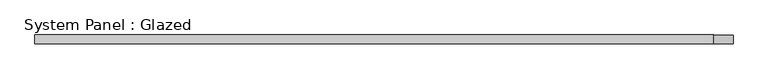
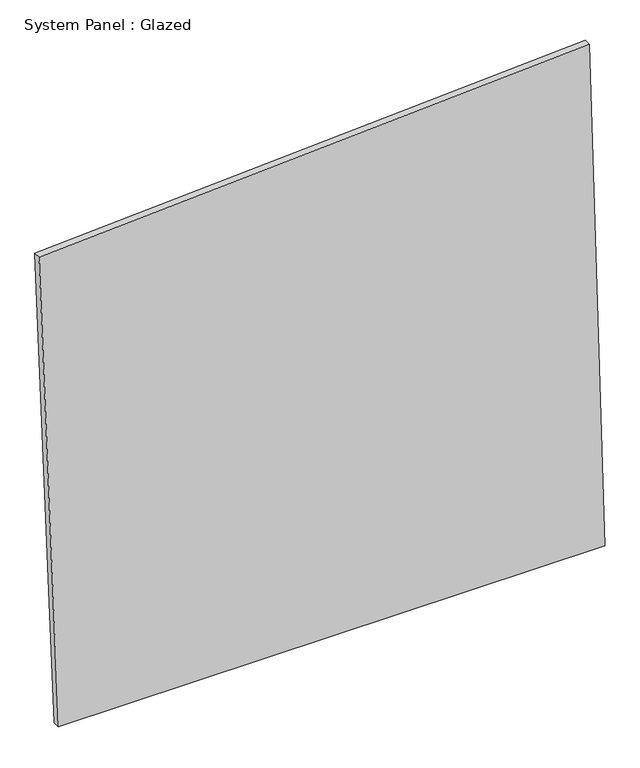
"""IFC4 building model written with IfcOpenShell, lengths in millimetres: plate geometry, System Panel : Glazed."""

import ifcopenshell
import ifcopenshell.guid

model = None  # the IFC model being written
_history = None  # IfcOwnerHistory: only IFC2X3 demands one
_inside = {}  # id of a spatial element -> (the spatial element, [elements in it])
_under = {}  # id of a project, library or spatial element -> (it, [spatial elements below it])
_declared = {}  # id of a project -> (the project, [libraries it declares])
_typed = {}  # id of a type object -> (the type object, [elements of that type])
_made_of = {}  # id of a material, layer set ... -> (it, [elements and type objects made of it])


def new_model(schema):
    """Start an empty IFC model of exactly this schema.

    Asked for "IFC4X3", IfcOpenShell would pick the latest addendum, in which some entities
    have other attributes; the version numbers below select the first issue.
    IFC2X3 requires an IfcOwnerHistory on every rooted entity: one is made here for all.
    """
    global model, _history
    if schema == "IFC4X3":
        model = ifcopenshell.file(schema_version=(4, 3, 0, 0))
    else:
        model = ifcopenshell.file(schema=schema)
    _inside.clear()
    _under.clear()
    _declared.clear()
    _typed.clear()
    _made_of.clear()
    _history = None
    if model.schema == "IFC2X3":
        org = make("IfcOrganization", Name="unknown")
        user = make(
            "IfcPersonAndOrganization",
            ThePerson=make("IfcPerson", FamilyName="unknown"),
            TheOrganization=org,
        )
        app = make(
            "IfcApplication",
            ApplicationDeveloper=org,
            Version="unknown",
            ApplicationFullName="unknown",
            ApplicationIdentifier="unknown",
        )
        _history = make(
            "IfcOwnerHistory",
            OwningUser=user,
            OwningApplication=app,
            ChangeAction="ADDED",
            CreationDate=0,
        )
    return model


def make(cls, **values):
    """One entity of the class cls with the attributes given. An attribute that is None is left unset."""
    return model.create_entity(
        cls, **{name: value for name, value in values.items() if value is not None}
    )


def rooted(cls, **values):
    """An entity with a GlobalId (a new one), such as an element, a storey or a relation."""
    return make(cls, GlobalId=ifcopenshell.guid.new(), OwnerHistory=_history, **values)


def si_unit(unit_type, name, prefix=None):
    """IfcSIUnit, for example si_unit("LENGTHUNIT", "METRE", prefix="MILLI")."""
    return make("IfcSIUnit", UnitType=unit_type, Prefix=prefix, Name=name)


def assignment(units):
    """IfcUnitAssignment: the units of a project."""
    return None if units is None else make("IfcUnitAssignment", Units=units)


def point(xyz):
    """IfcCartesianPoint."""
    return None if xyz is None else make("IfcCartesianPoint", Coordinates=xyz)


def direction(xyz):
    """IfcDirection."""
    return None if xyz is None else make("IfcDirection", DirectionRatios=xyz)


def frame(location, z_axis=None, x_axis=None):
    """IfcAxis2Placement3D, a coordinate frame: its origin and axes. An axis left out is left unset."""
    return make(
        "IfcAxis2Placement3D",
        Location=point(location),
        Axis=direction(z_axis),
        RefDirection=direction(x_axis),
    )


def origin():
    """The frame at (0, 0, 0) with its axes left unset."""
    return frame((0.0, 0.0, 0.0))


def place(relative_to, where):
    """IfcLocalPlacement: puts the frame where relative to a parent placement (None: the world)."""
    return make(
        "IfcLocalPlacement", PlacementRelTo=relative_to, RelativePlacement=where
    )


def context(
    kind, dimensions, precision=None, world=None, true_north=None, identifier=None
):
    """IfcGeometricRepresentationContext, for example the 3D "Model" context."""
    return make(
        "IfcGeometricRepresentationContext",
        ContextIdentifier=identifier,
        ContextType=kind,
        CoordinateSpaceDimension=dimensions,
        Precision=precision,
        WorldCoordinateSystem=world,
        TrueNorth=true_north,
    )


def project(units=None, contexts=None):
    """IfcProject with its units and contexts."""
    return rooted(
        "IfcProject",
        Name="project",
        RepresentationContexts=contexts,
        UnitsInContext=assignment(units),
    )


def spatial(cls, under=None, at=None, **own):
    """A site, building, storey or space (cls), placed at a placement, below another one or the project."""
    s = rooted(cls, ObjectPlacement=at, **own)
    if under is not None:
        _under.setdefault(under.id(), (under, []))[1].append(s)
    return s


def polyline(points):
    """IfcPolyline through the points."""
    return make("IfcPolyline", Points=[point(p) for p in points])


def outline(outer, holes=None, kind="AREA"):
    """IfcArbitraryClosedProfileDef: a profile drawn as a closed curve; with holes, ...WithVoids."""
    if holes is None:
        return make("IfcArbitraryClosedProfileDef", ProfileType=kind, OuterCurve=outer)
    return make(
        "IfcArbitraryProfileDefWithVoids",
        ProfileType=kind,
        OuterCurve=outer,
        InnerCurves=holes,
    )


def extrude(swept, where, along, depth):
    """IfcExtrudedAreaSolid: the profile swept, set in the frame where, extruded along a direction by depth."""
    return make(
        "IfcExtrudedAreaSolid",
        SweptArea=swept,
        Position=where,
        ExtrudedDirection=direction(along),
        Depth=depth,
    )


def shape(context_of_items, identifier, shape_type, items):
    """IfcShapeRepresentation: the items that make up one representation, for example the "Body"."""
    return make(
        "IfcShapeRepresentation",
        ContextOfItems=context_of_items,
        RepresentationIdentifier=identifier,
        RepresentationType=shape_type,
        Items=items,
    )


def source(mapping_origin, context_of_items, identifier, shape_type, items):
    """IfcRepresentationMap: a shape defined once, which mapped items show again and again."""
    return make(
        "IfcRepresentationMap",
        MappingOrigin=mapping_origin,
        MappedRepresentation=shape(context_of_items, identifier, shape_type, items),
    )


def transform(
    local_origin,
    x_axis=None,
    y_axis=None,
    z_axis=None,
    scale=None,
    scale2=None,
    scale3=None,
    uniform=True,
):
    """IfcCartesianTransformationOperator3D, or its non-uniform kind. x_axis, y_axis, z_axis: its Axis1, 2, 3."""
    if uniform:
        return make(
            "IfcCartesianTransformationOperator3D",
            Axis1=direction(x_axis),
            Axis2=direction(y_axis),
            LocalOrigin=point(local_origin),
            Scale=scale,
            Axis3=direction(z_axis),
        )
    return make(
        "IfcCartesianTransformationOperator3DnonUniform",
        Axis1=direction(x_axis),
        Axis2=direction(y_axis),
        LocalOrigin=point(local_origin),
        Scale=scale,
        Axis3=direction(z_axis),
        Scale2=scale2,
        Scale3=scale3,
    )


def mapped(mapping_source, mapping_target):
    """IfcMappedItem: shows the shape of a source again, moved by a transform."""
    return make(
        "IfcMappedItem", MappingSource=mapping_source, MappingTarget=mapping_target
    )


def made_of(thing, what):
    """Note that an element or type object is made of a material, layer set ...; save() writes the relation."""
    if what is not None:
        _made_of.setdefault(what.id(), (what, []))[1].append(thing)
    return thing


def element(
    cls,
    number,
    at=None,
    inside=None,
    cuts=None,
    type_object=None,
    material=None,
    context=None,
    identifier="Body",
    shape_type=None,
    held_by="IfcProductDefinitionShape",
    body=None,
    shapes=None,
    **own,
):
    """One element of the class cls, such as IfcWall. Its Tag is "e" and its number.

    at: its placement. inside: the storey or other place that contains it. cuts: it is an
    opening in that element (IfcRelVoidsElement). A single representation is given by context,
    identifier, shape_type and body (its items); several are given by shapes. held_by: the class
    of the entity that holds the representations. save() writes the other relations.
    """
    e = rooted(cls, Tag="e%d" % number, ObjectPlacement=at, **own)
    if body is not None:
        shapes = [shape(context, identifier, shape_type, body)]
    if shapes is not None:
        e.Representation = make(held_by, Representations=shapes)
    if inside is not None:
        _inside.setdefault(inside.id(), (inside, []))[1].append(e)
    if cuts is not None:
        rooted(
            "IfcRelVoidsElement", RelatingBuildingElement=cuts, RelatedOpeningElement=e
        )
    if type_object is not None:
        _typed.setdefault(type_object.id(), (type_object, []))[1].append(e)
    return made_of(e, material)


def aggregate(whole, parts):
    """IfcRelAggregates: a whole, such as a stair, and the parts it consists of."""
    return rooted("IfcRelAggregates", RelatingObject=whole, RelatedObjects=parts)


def save(model, path):
    """Write the relations noted so far, then the file.

    IfcRelAggregates (storeys below a building ...), IfcRelContainedInSpatialStructure (elements
    in a storey), IfcRelDefinesByType, IfcRelAssociatesMaterial and IfcRelDeclares: one each for
    every whole, place, type object, material and project.
    """
    for whole, parts in _under.values():
        aggregate(whole, parts)
    for where, things in _inside.values():
        rooted(
            "IfcRelContainedInSpatialStructure",
            RelatedElements=things,
            RelatingStructure=where,
        )
    for kind, things in _typed.values():
        rooted("IfcRelDefinesByType", RelatedObjects=things, RelatingType=kind)
    for what, things in _made_of.values():
        rooted("IfcRelAssociatesMaterial", RelatedObjects=things, RelatingMaterial=what)
    for by, libraries in _declared.values():
        rooted("IfcRelDeclares", RelatingContext=by, RelatedDefinitions=libraries)
    model.write(path)


def system_panel_glazed_ae3b4f36(model_context):
    return source(origin(), model_context, "Body", "SweptSolid", [
        extrude(outline(polyline([(0.0, -923.1075404), (0.0, 991.2413385), (1874.9756018, 936.3989323), (1761.0780772, -991.2413385), (0.0, -923.1075404)])), frame((0.0, -49.5, 0.0), z_axis=(0.0, 1.0, 0.0), x_axis=(0.0, 0.0, 1.0)), (0.0, 0.0, 1.0), 25.0),
    ])


if __name__ == "__main__":
    model = new_model("IFC4")
    model_context = context("Model", 3, world=origin())
    ifc_project = project(units=[si_unit("LENGTHUNIT", "METRE", prefix="MILLI")], contexts=[model_context])
    site = spatial("IfcSite", under=ifc_project)
    building = spatial("IfcBuilding", under=site)
    placement = place(None, origin())
    system_panel_glazed_shape = system_panel_glazed_ae3b4f36(model_context)
    element("IfcPlate", 1, ObjectType="System Panel : Glazed", at=placement, inside=building, context=model_context, shape_type="MappedRepresentation", body=[
        mapped(system_panel_glazed_shape, transform((0.0, 0.0, 0.0), x_axis=(1.0, 0.0, 0.0), y_axis=(0.0, 1.0, 0.0), z_axis=(0.0, 0.0, 1.0))),
    ])
    save(model, "model.ifc")

# Revit data of these elements
# Element 1 (IfcPlate, "System Panel : Glazed")
#   Materials on its faces: "Glass, Clear Glazing"
# Materials
#   "Glass, Clear Glazing": class "Glass", colour RGB 247 249 248, transparency 0.85, Description = "Clear glazing", Cost = 0
